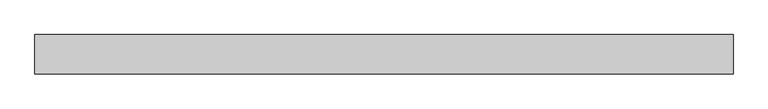
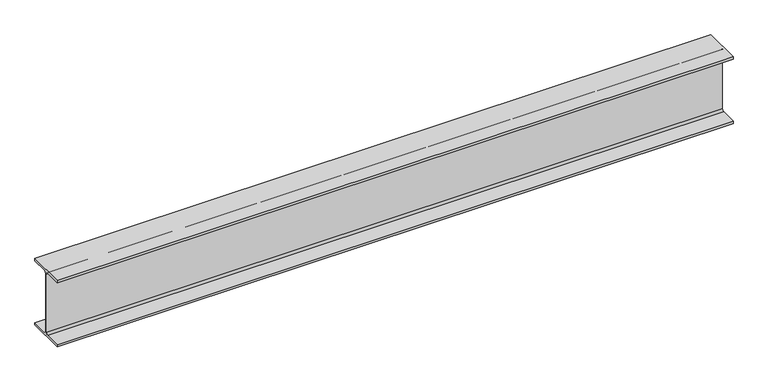
"""IFC4 building model written with IfcOpenShell, lengths in millimetres: beam geometry, Old_Steel Beam_H-KSD3502 : H_SB_ASB_H-250×125x6x9."""

from ifc_helpers import new_model, si_unit, point, frame, frame_2d, origin, place, context, project, spatial, polyline, circle_curve, trimmed, segment, composite_curve, outline, extrude, source, transform, mapped, element, save


def beam_201670e7(model_context):
    return source(origin(), model_context, "Body", "SweptSolid", [
        extrude(outline(composite_curve([segment(polyline([(82.5, -141.5), (82.5, -151.7), (-82.5, -151.7), (-82.5, -141.5), (-11.9, -141.5)]), True, "CONTINUOUS"), segment(trimmed(circle_curve(frame_2d((-11.9, -132.6)), 8.9), [point((-11.9, -141.5))], [point((-3.0, -132.6))], True, "CARTESIAN"), True, "CONTINUOUS"), segment(polyline([(-3.0, -132.6), (-3.0, 132.6)]), True, "CONTINUOUS"), segment(trimmed(circle_curve(frame_2d((-11.9, 132.6)), 8.9), [point((-3.0, 132.6))], [point((-11.9, 141.5))], True, "CARTESIAN"), True, "CONTINUOUS"), segment(polyline([(-11.9, 141.5), (-82.5, 141.5), (-82.5, 151.7), (82.5, 151.7), (82.5, 141.5), (11.9, 141.5)]), True, "CONTINUOUS"), segment(trimmed(circle_curve(frame_2d((11.9, 132.6)), 8.9), [point((11.9, 141.5))], [point((3.0, 132.6))], True, "CARTESIAN"), True, "CONTINUOUS"), segment(polyline([(3.0, 132.6), (3.0, -132.6)]), True, "CONTINUOUS"), segment(trimmed(circle_curve(frame_2d((11.9, -132.6)), 8.9), [point((3.0, -132.6))], [point((11.9, -141.5))], True, "CARTESIAN"), True, "CONTINUOUS"), segment(polyline([(11.9, -141.5), (82.5, -141.5)]), True, "CONTINUOUS")], self_intersect=False)), frame((-1529.8, 0.0, 0.0), z_axis=(1.0, 0.0, 0.0), x_axis=(0.0, 1.0, 0.0)), (0.0, 0.0, 1.0), 2912.1488581),
    ])


if __name__ == "__main__":
    model = new_model("IFC4")
    model_context = context("Model", 3, world=origin())
    ifc_project = project(units=[si_unit("LENGTHUNIT", "METRE", prefix="MILLI")], contexts=[model_context])
    site = spatial("IfcSite", under=ifc_project)
    building = spatial("IfcBuilding", under=site)
    placement = place(None, origin())
    beam_shape = beam_201670e7(model_context)
    element("IfcBeam", 1, ObjectType="Old_Steel Beam_H-KSD3502 : H_SB_ASB_H-250×125x6x9", at=placement, inside=building, context=model_context, shape_type="MappedRepresentation", body=[
        mapped(beam_shape, transform((0.0, 0.0, 0.0), x_axis=(1.0, 0.0, 0.0), y_axis=(0.0, 1.0, 0.0), z_axis=(0.0, 0.0, 1.0))),
    ])
    save(model, "model.ifc")

# Revit data of these elements
# Type "Old_Steel Beam_H-KSD3502 : H_SB_ASB_H-250×125x6x9"
#   Width = 12.5 cm
#   Web Thickness = 0.6 cm
#   Web Fillet = 1.2 cm
#   Warping Constant = 42539.8 cm⁶
#   Torsional Moment of Inertia = 7.8102 cm⁴
#   Torsional Modulus = 1.0 cm³
#   Section Area = 37.66 cm²
#   Plastic Modulus weak axis = 73.1 cm³
#   Plastic Modulus strong axis = 366.0 cm³
#   Perimeter = 0.97 m²/m
#   Nominal Weight = 29.60 kgf/m
#   Moment of Inertia weak axis = 294.00 cm⁴
#   Moment of Inertia strong axis = 4050.00 cm⁴
#   Height = 25.0 cm
#   Flange Thickness = 0.9 cm
#   Elastic Modulus weak axis = 47.0 cm³
#   Elastic Modulus strong axis = 324.0 cm³
#   Centroid Vertical = 12.5 cm
#   Centroid Horizontal = 6.25 cm
#   Length [instance default] = 1.5240 m
#   Structural Material [instance default] = Steel, 45-345
#   Assembly Code = ""
# Element 1 (IfcBeam, "Old_Steel Beam_H-KSD3502 : H_SB_ASB_H-250×125x6x9")
#   Structural Material = none
# Materials
#   "Steel, 45-345": class "Metal", colour RGB 189 187 185, transparency 0, Description = "Steel 345 MPa", Cost = 0
